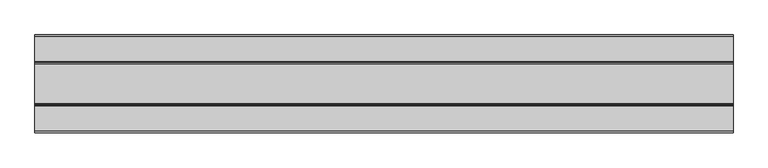
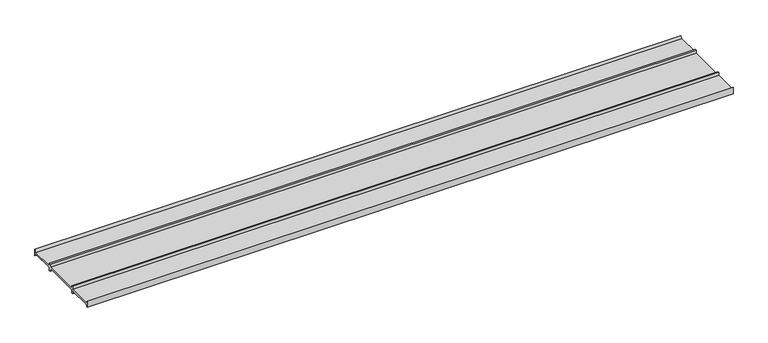
"""IFC4 building model written with IfcOpenShell, lengths in millimetres: proxy geometry, TN_Гидрошпонка ТН Фундамент : Гидрошпонка ТН Фундамент ТШ-В-210."""

from ifc_helpers import new_model, si_unit, frame, origin, place, context, project, spatial, polyline, outline, extrude, source, transform, mapped, element, save


def specialty_equipment_78d658e4(model_context):
    return source(origin(), model_context, "Body", "SweptSolid", [
        extrude(outline(polyline([(-43.5006268, -7.0044352), (-46.4993732, -7.0044352), (-47.7344441, 0.0), (-101.5809483, 0.0), (-105.0, -5.5044352), (-105.0, 9.4955648), (-101.5809483, 3.9911296), (-47.7344441, 3.9911296), (-46.4993732, 10.9955648), (-43.5006268, 10.9955648), (-42.2655559, 3.9911296), (42.2655559, 3.9911296), (43.5006268, 10.9955648), (46.4993732, 10.9955648), (47.7344441, 3.9911296), (101.5809483, 3.9911296), (105.0, 9.4955648), (105.0, -5.5044352), (101.5809483, 0.0), (47.7344441, 0.0), (46.4993732, -7.0044352), (43.5006268, -7.0044352), (42.2655559, 0.0), (-42.2655559, 0.0), (-43.5006268, -7.0044352)])), frame((0.0, 0.0, 0.0), z_axis=(1.0, 0.0, 0.0), x_axis=(0.0, 1.0, 0.0)), (0.0, 0.0, 1.0), 1500.0),
    ])


if __name__ == "__main__":
    model = new_model("IFC4")
    model_context = context("Model", 3, world=origin())
    ifc_project = project(units=[si_unit("LENGTHUNIT", "METRE", prefix="MILLI")], contexts=[model_context])
    site = spatial("IfcSite", under=ifc_project)
    building = spatial("IfcBuilding", under=site)
    placement = place(None, origin())
    specialty_equipment_shape = specialty_equipment_78d658e4(model_context)
    element("IfcBuildingElementProxy", 1, Name="TN_Гидрошпонка ТН Фундамент : Гидрошпонка ТН Фундамент ТШ-В-210", ObjectType="TN_Гидрошпонка ТН Фундамент : Гидрошпонка ТН Фундамент ТШ-В-210", at=placement, inside=building, context=model_context, shape_type="MappedRepresentation", body=[
        mapped(specialty_equipment_shape, transform((0.0, 0.0, 0.0), x_axis=(1.0, 0.0, 0.0), y_axis=(0.0, 1.0, 0.0), z_axis=(0.0, 0.0, 1.0))),
    ])
    save(model, "model.ifc")

# Revit data of these elements
# Type "TN_Гидрошпонка ТН Фундамент : Гидрошпонка ТН Фундамент ТШ-В-210"
#   Description = "Внутренние гидроизоляционные шпонки ТН Фундамент ТШ-В предназначены для герметизации технологических швов бетонирования при строительстве подземных и заглубленных конструкций зданий и сооружений различного назначения и класса ответственности."
#   Type Comments = "п.м."
#   Manufacturer = "ТехноНИКОЛЬ"
#   URL = "https://nav.tn.ru/catalog/gidroizolyatsiya/komplektatsiya-dlya-gidroizolyatsii/gidroshponki-tekhnonikol-fundament-tsh-v/"
#   ADSK_Примечание = ""
#   ADSK_Обозначение [instance default] = "ТехноНИКОЛЬ"
#   ADSK_Наименование = "Гидрошпонка ТН Фундамент ТШ-В-210"
#   ADSK_Масса_Текст = ""
#   ADSK_Марка = ""
#   ADSK_Код изделия = "66674"
#   ADSK_Завод-изготовитель [instance default] = "ТехноНИКОЛЬ"
#   ADSK_Единица измерения [instance default] = "п.м."
#   ADSK_Группирование = "Гидрошпонки"
#   ADSK_URL страницы изделия = "https://nav.tn.ru/catalog/gidroizolyatsiya/komplektatsiya-dlya-gidroizolyatsii/gidroshponki-tekhnonikol-fundament-tsh-v/"
#   ADSK_URL документации изделия = "https://nav.tn.ru/upload/iblock/a6b/ewrhpb0y1xrl8jlgtx64kildvudhcq55/Tekhlist-7.401_Gidroshponki-TN-Fundament-TSH_V_RU_ru.pdf"
#   built-in parameter 1001306 [instance default] = 3.28084 (stored number, unit not read)
#   ADSK_Размер_Длина [instance default] = 1000 mm
#   ADSK_Количество [instance default] = 1
#   Гидрошпонка ТН Фундамент ТШ-Н-210 = no
#   Гидрошпонка ТН Фундамент ДШП-В-50 = no
#   Гидрошпонка ТН Фундамент ДШП-В-20 = no
#   Гидрошпонка ТН Фундамент ДШ-В-280 = no
#   Гидрошпонка ТН Фундамент ДШ-В-250 = no
#   Гидрошпонка ТН Фундамент ТШ-В-250 = no
#   Гидрошпонка ТН Фундамент ТПС-В 140-1 = no
#   Гидрошпонка ТН Фундамент ДШ-Н-280 = no
#   Гидрошпонка ТН Фундамент ДШ-Н-250 = no
#   Гидрошпонка ТН Фундамент ТПС-В 100-2 = no
#   Гидрошпонка ТН Фундамент ТШ-Н-250 = no
#   Гидрошпонка ТН Фундамент ТШ-В-210 = yes
#   Материал = TN_ПВХ_Черный
#   Default Elevation = 0
# Element 1 (IfcBuildingElementProxy, "TN_Гидрошпонка ТН Фундамент : Гидрошпонка ТН Фундамент ТШ-В-210")
#   built-in parameter 1001306 = 4.92126 (stored number, unit not read)
#   ADSK_Размер_Длина = 1500 mm
#   ADSK_Количество = 1.5
#   Materials on its faces: "TN_ПВХ_Черный"
# Materials
#   "TN_ПВХ_Черный": class "Типовые", colour RGB 48 48 48, transparency 0, Cost = 0
